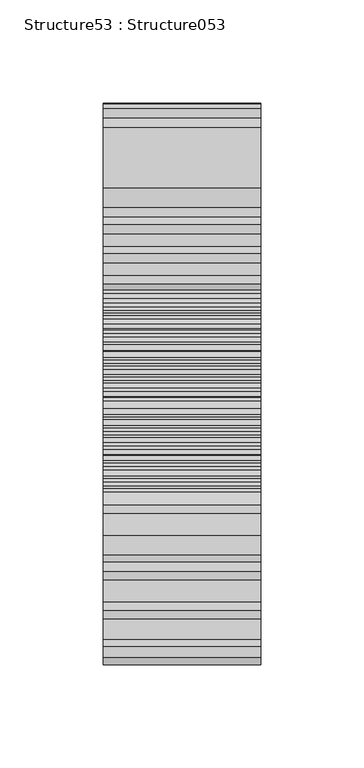
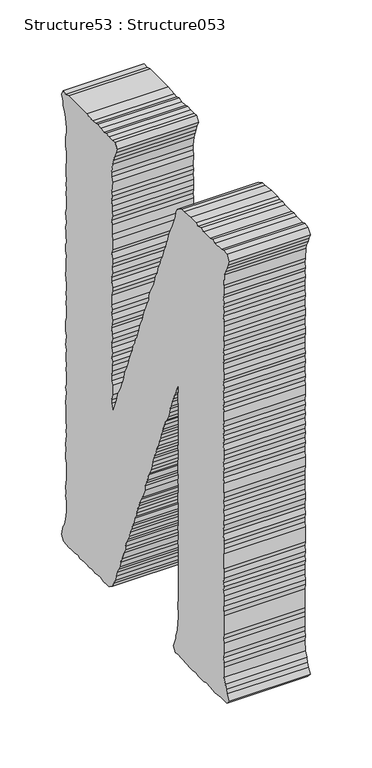
"""IFC4 building model written with IfcOpenShell, lengths in millimetres: proxy geometry, Structure53 : Structure053."""

from ifc_helpers import new_model, si_unit, frame, origin, place, context, project, spatial, polyline, outline, extrude, source, transform, mapped, element, save


def structure53_structure053_f29fcba1(model_context):
    return source(origin(), model_context, "Body", "SweptSolid", [
        extrude(outline(polyline([(256849.9794414, 3575.0851816), (256851.717228, 3569.2524442), (256852.3189547, 3565.7094775), (256855.839457, 3556.3417965), (256852.8982169, 3551.0658569), (256848.2175856, 3551.6675836), (256843.5385589, 3551.0658569), (256833.5755696, 3551.0658569), (256830.0550673, 3550.4833855), (256824.7727093, 3550.4833855), (256820.6954093, 3551.0658569), (256815.4130513, 3550.4833855), (256806.610191, 3550.4833855), (256802.508822, 3551.6675836), (256796.6696662, 3551.6675836), (256793.1266995, 3550.4833855), (256788.4685326, 3550.4833855), (256779.0864101, 3551.6675836), (256769.7042876, 3551.6675836), (256766.2046452, 3555.7416744), (256769.102561, 3561.025637), (256770.2835499, 3565.1254015), (256771.4645388, 3569.2524442), (256773.8040521, 3574.5107332), (256774.4057788, 3584.4689087), (256773.8040521, 3589.1527492), (256774.9866456, 3593.2541183), (256774.4057788, 3597.9540049), (256774.4057788, 3607.8961343), (256774.9866456, 3612.0135494), (256774.4057788, 3616.69739), (256774.4057788, 3635.4407751), (256773.8040521, 3640.114988), (256773.8040521, 3644.8245022), (256774.4057788, 3649.5003197), (256774.4057788, 3654.7842823), (256774.9866456, 3659.4584952), (256773.8040521, 3664.1423357), (256774.9866456, 3667.6853024), (256773.8040521, 3672.9435914), (256774.4057788, 3678.2018803), (256773.8040521, 3682.3289231), (256773.8040521, 3696.9709391), (256774.4057788, 3701.6547796), (256774.4057788, 3706.3289925), (256773.8040521, 3709.8559132), (256774.9866456, 3715.7143242), (256774.9866456, 3719.2316172), (256773.8040521, 3725.0996559), (256773.8040521, 3729.7738688), (256774.4057788, 3733.8736333), (256774.9866456, 3739.1592005), (256774.4057788, 3743.8414364), (256774.9866456, 3747.9428055), (256774.4057788, 3752.04257), (256773.8040521, 3757.3185096), (256773.8040521, 3766.684586), (256774.9866456, 3771.3860772), (256774.9866456, 3776.0618947), (256773.8040521, 3780.7441306), (256774.9866456, 3784.8438951), (256773.8040521, 3790.7039107), (256774.4057788, 3794.2292268), (256773.8040521, 3798.9050443), (256774.9866456, 3804.1890069), (256773.8040521, 3809.4729695), (256774.9866456, 3812.9726119), (256773.8040521, 3818.2309008), (256774.9866456, 3822.348316), (256773.8040521, 3828.2163546), (256773.8040521, 3837.6000817), (256774.9866456, 3841.6741725), (256773.8040521, 3846.3772683), (256774.9866456, 3851.0595042), (256774.9866456, 3855.1769193), (256773.8040521, 3861.0192843), (256774.9866456, 3865.7015202), (256773.8040521, 3869.2444869), (256774.4057788, 3873.9203044), (256774.9866456, 3879.1769888), (256774.9866456, 3884.4609514), (256773.8040521, 3888.5623205), (256773.8040521, 3893.822214), (256774.9866456, 3897.3475301), (256774.4057788, 3902.6314927), (256773.8040521, 3907.3313793), (256773.8040521, 3912.5896682), (256774.4057788, 3916.0909152), (256774.4057788, 3921.9733953), (256773.8040521, 3926.6492128), (256774.9866456, 3931.3346579), (256774.4057788, 3936.0345445), (256774.9866456, 3940.1166583), (256773.8040521, 3944.8165449), (256774.9866456, 3950.0940891), (256773.8040521, 3953.5937315), (256774.4057788, 3959.4617701), (256773.8040521, 3962.9774586), (256773.2247899, 3973.5197101), (256772.043801, 3977.6194746), (256769.102561, 3982.8793681), (256767.966501, 3986.4046842), (256766.2046452, 3991.0788971), (256769.7042876, 3996.390138), (256774.9866456, 3996.9645864), (256778.4846834, 3995.7803883), (256788.4685326, 3995.7803883), (256792.5474372, 3996.9645864), (256796.6696662, 3995.7803883), (256807.1894533, 3995.7803883), (256811.3116822, 3996.9645864), (256815.9923135, 3995.7803883), (256819.5144204, 3996.9645864), (256828.8965429, 3996.9645864), (256839.4371898, 3995.7803883), (256843.5385589, 3995.7803883), (256849.9794414, 3992.2614906), (256851.717228, 3988.7634528), (256852.8982169, 3982.8793681), (256854.6584681, 3978.8036727), (256856.4203238, 3974.7055128), (256857.6013127, 3971.1785921), (256860.5200883, 3966.5043792), (256862.2803394, 3961.2204166), (256864.0421952, 3957.1190475), (256865.2231841, 3952.9920048), (256867.540233, 3947.7337158), (256868.1419596, 3944.235678), (256870.481473, 3939.5325823), (256872.2433287, 3934.8503464), (256873.9811154, 3930.1745289), (256876.3430932, 3926.6492128), (256877.5240821, 3922.5494483), (256879.2859379, 3917.8479571), (256881.046189, 3914.3499193), (256882.2047134, 3909.0627475), (256885.123489, 3904.9645876), (256886.3060825, 3900.8648231), (256887.4870714, 3895.5888836), (256890.405847, 3890.905043), (256893.9279539, 3883.2863809), (256895.688205, 3879.1769888), (256896.2674672, 3874.5043805), (256898.6069806, 3869.8189354), (256900.3672317, 3864.5446004), (256902.7083497, 3860.4432313), (256903.8893386, 3857.5019912), (256905.6271253, 3851.6612309), (256906.8081142, 3848.7167816), (256909.1716966, 3844.0345457), (256910.9319477, 3838.7586061), (256912.0680077, 3834.6588416), (256913.8507233, 3830.5574726), (256915.0092477, 3825.2911606), (256917.9520924, 3822.348316), (256918.5313546, 3817.6741031), (256921.4501302, 3813.5743386), (256922.6311191, 3808.290376), (256924.9947015, 3803.5872802), (256926.7324882, 3799.5051664), (256928.4927393, 3795.4037973), (256929.0720015, 3791.8865042), (256931.435584, 3786.0280932), (256933.7750973, 3781.9299333), (256935.512884, 3777.8285642), (256936.6938729, 3773.11905), (256937.8748618, 3768.4432325), (256939.6367175, 3764.9435901), (256941.3969687, 3760.2437036), (256943.7140176, 3755.559863), (256946.0776, 3752.04257), (256948.4171133, 3743.2332913), (256950.1549, 3739.1592005), (256952.5168778, 3733.2991849), (256954.2787336, 3729.1737467), (256955.4597225, 3730.3563402), (256956.5957825, 3735.0578314), (256956.5957825, 3738.5574738), (256955.4597225, 3744.4158848), (256955.4597225, 3753.8012165), (256956.5957825, 3757.3185096), (256956.5957825, 3762.5848215), (256956.0389847, 3767.2590344), (256956.0389847, 3772.5606477), (256955.4597225, 3777.2444882), (256956.5957825, 3780.7441306), (256955.4597225, 3785.4456218), (256956.5957825, 3790.1294623), (256956.5957825, 3794.8309535), (256955.4597225, 3800.0876378), (256956.0389847, 3804.1890069), (256956.5957825, 3810.0474179), (256956.0389847, 3813.5743386), (256955.4597225, 3818.2309008), (256956.5957825, 3823.5341187), (256956.0389847, 3828.2163546), (256956.5957825, 3832.8921721), (256956.5957825, 3842.2758992), (256955.4597225, 3846.9757858), (256955.4597225, 3850.4754282), (256956.5957825, 3856.3161885), (256956.5957825, 3859.8591552), (256955.4597225, 3864.5446004), (256956.0389847, 3870.4030114), (256955.4597225, 3873.9203044), (256955.4597225, 3878.5784713), (256956.5957825, 3884.4609514), (256955.4597225, 3887.9621984), (256955.4597225, 3897.3475301), (256956.0389847, 3903.2059411), (256956.0389847, 3912.5896682), (256956.5957825, 3916.6653636), (256955.4597225, 3921.3748778), (256956.0389847, 3925.4746423), (256956.0389847, 3930.7329312), (256956.5957825, 3936.0345445), (256956.0389847, 3940.718385), (256956.5957825, 3944.235678), (256955.4597225, 3954.7506513), (256956.5957825, 3959.4617701), (256956.5957825, 3964.1343784), (256954.8579958, 3972.9372387), (256953.0977447, 3978.2035506), (256951.9151511, 3982.3225704), (256949.5756378, 3987.5792547), (256947.8378511, 3992.2614906), (256950.7566267, 3997.5486624), (256954.8579958, 3996.9645864), (256960.719616, 3996.9645864), (256965.3986427, 3997.5486624), (256968.9207496, 3996.390138), (256974.7807652, 3996.390138), (256979.4613965, 3997.5486624), (256982.9835034, 3996.390138), (256987.6625301, 3996.390138), (256997.0446526, 3997.5486624), (257026.3286846, 3997.5486624), (257031.0317804, 3996.390138), (257035.7124117, 3996.9645864), (257037.4726629, 3992.2614906), (257035.7124117, 3986.4046842), (257035.1331495, 3982.8793681), (257032.7695671, 3977.6194746), (257031.0317804, 3972.9372387), (257029.873256, 3962.9774586), (257029.873256, 3959.4617701), (257031.0317804, 3953.5937315), (257031.0317804, 3944.8165449), (257029.873256, 3940.1166583), (257029.873256, 3930.1745289), (257030.4525182, 3926.6492128), (257030.4525182, 3916.6653636), (257029.873256, 3912.0071968), (257030.4525182, 3907.3313793), (257029.873256, 3903.2059411), (257030.4525182, 3898.5301236), (257029.873256, 3893.246161), (257029.873256, 3883.8881076), (257031.0317804, 3879.1769888), (257029.873256, 3869.8189354), (257031.0317804, 3865.1190488), (257030.4525182, 3859.8591552), (257030.4525182, 3855.7353217), (257029.873256, 3850.4754282), (257031.0317804, 3846.9757858), (257031.0317804, 3841.0900965), (257029.873256, 3836.9919366), (257030.4525182, 3832.3161191), (257030.4525182, 3822.348316), (257031.0317804, 3818.2309008), (257030.4525182, 3812.9726119), (257029.873256, 3809.4729695), (257029.873256, 3804.7730829), (257030.4525182, 3799.5051664), (257029.873256, 3795.4037973), (257030.4525182, 3790.1294623), (257029.873256, 3784.8438951), (257029.873256, 3775.4874463), (257031.0317804, 3771.3860772), (257031.0317804, 3762.0023501), (257029.873256, 3757.8753073), (257030.4525182, 3752.04257), (257031.0317804, 3748.5429276), (257029.873256, 3743.8414364), (257030.4525182, 3739.1592005), (257030.4525182, 3734.47536), (257029.873256, 3728.5992983), (257030.4525182, 3725.0996559), (257029.873256, 3719.2316172), (257029.873256, 3709.8559132), (257031.0317804, 3705.7545441), (257029.873256, 3701.6547796), (257030.4525182, 3695.786741), (257031.0317804, 3691.0868544), (257030.4525182, 3687.0127636), (257030.4525182, 3672.3691429), (257029.873256, 3668.2437048), (257030.4525182, 3662.9854159), (257029.873256, 3659.4584952), (257030.4525182, 3653.6000842), (257031.0317804, 3650.1004418), (257030.4525182, 3644.2420307), (257031.0317804, 3640.114988), (257031.0317804, 3635.4407751), (257029.873256, 3631.3410106), (257029.873256, 3616.69739), (257030.4525182, 3611.4134274), (257031.0317804, 3607.3393366), (257030.4525182, 3602.0280957), (257031.0317804, 3598.5284533), (257029.873256, 3593.2541183), (257029.873256, 3583.2863152), (257031.0317804, 3575.0851816), (257032.7695671, 3569.2524442), (257035.1331495, 3565.7094775), (257036.8934006, 3559.8671125), (257038.0743895, 3556.3417965), (257034.5522827, 3551.0658569), (257030.4525182, 3551.0658569), (257026.3286846, 3550.4833855), (257020.4911335, 3551.0658569), (257016.3897644, 3551.0658569), (257011.1074064, 3551.6675836), (257007.6093686, 3550.4833855), (257001.7252839, 3551.0658569), (256998.2272461, 3551.0658569), (256992.3656259, 3550.4833855), (256988.2417923, 3551.6675836), (256983.5627656, 3550.4833855), (256978.3028721, 3551.6675836), (256974.7807652, 3551.6675836), (256970.1017385, 3550.4833855), (256964.8193805, 3551.0658569), (256960.719616, 3551.0658569), (256954.8579958, 3555.1848766), (256953.0977447, 3559.2669905), (256950.1549, 3563.9412034), (256949.5756378, 3568.0682461), (256947.8378511, 3573.3265351), (256945.4758733, 3577.4535778), (256943.1347553, 3581.5276686), (256941.9537664, 3586.8116312), (256939.6367175, 3591.5131224), (256936.1146107, 3599.7126514), (256934.3318951, 3603.7963698), (256933.7750973, 3607.3393366), (256932.0148462, 3613.1720739), (256930.2529905, 3616.69739), (256927.3117504, 3621.3732075), (256926.7324882, 3625.472972), (256924.3929748, 3630.1824862), (256922.6311191, 3634.2822506), (256920.2916057, 3638.3563415), (256919.6898791, 3643.6579547), (256917.3728302, 3647.1575971), (256915.0092477, 3651.8590883), (256914.4299855, 3655.9428067), (256912.0680077, 3660.6250426), (256910.9319477, 3664.1423357), (256909.1716966, 3668.8261762), (256906.2288519, 3672.9435914), (256902.7083497, 3681.7271964), (256902.1290875, 3686.4030139), (256899.7879695, 3691.0868544), (256898.0277184, 3694.6298211), (256896.8467295, 3700.4705815), (256895.1089428, 3703.4134261), (256892.7453604, 3708.087639), (256890.9851092, 3712.7971532), (256890.405847, 3716.8985223), (256888.6680603, 3722.1568112), (256886.9078092, 3725.6741043), (256884.5442268, 3730.3563402), (256883.3632379, 3733.8736333), (256880.4444623, 3739.1592005), (256879.8652001, 3743.8414364), (256877.5240821, 3748.5429276), (256876.3430932, 3752.6170184), (256873.9811154, 3757.3185096), (256872.8450554, 3760.2437036), (256870.481473, 3766.1021146), (256869.3004841, 3770.2018791), (256866.404173, 3773.7015215), (256864.6439218, 3777.8285642), (256862.8596016, 3782.5027771), (256861.7010772, 3787.2042683), (256860.5200883, 3790.7039107), (256858.7823016, 3795.960595), (256855.839457, 3800.6717138), (256854.6584681, 3804.7730829), (256852.8982169, 3808.290376), (256851.1604303, 3812.9726119), (256848.8193123, 3817.6741031), (256847.6383234, 3818.2309008), (256848.2175856, 3812.9726119), (256848.8193123, 3808.8888934), (256848.8193123, 3803.0064134), (256848.2175856, 3798.9050443), (256847.6383234, 3794.2292268), (256848.2175856, 3790.1294623), (256848.2175856, 3780.7441306), (256847.6383234, 3774.8857196), (256847.6383234, 3766.684586), (256848.2175856, 3760.818152), (256848.8193123, 3757.3185096), (256848.2175856, 3752.6170184), (256847.6383234, 3747.3587295), (256848.8193123, 3742.6748889), (256848.8193123, 3732.7167134), (256848.2175856, 3728.0152223), (256848.8193123, 3723.9154578), (256848.2175856, 3718.6571688), (256847.6383234, 3714.5301261), (256848.8193123, 3709.8559132), (256848.8193123, 3704.5879966), (256848.2175856, 3700.4705815), (256847.6383234, 3696.3884676), (256847.6383234, 3691.6869765), (256848.2175856, 3687.587212), (256848.2175856, 3681.7271964), (256848.8193123, 3677.0449605), (256848.2175856, 3672.3691429), (256847.6383234, 3668.2437048), (256848.8193123, 3663.5598643), (256847.6383234, 3658.3015753), (256847.6383234, 3648.9258713), (256848.2175856, 3644.8245022), (256848.2175856, 3635.4407751), (256847.6383234, 3631.3410106), (256847.6383234, 3611.4134274), (256848.2175856, 3607.3393366), (256848.8193123, 3602.0280957), (256848.8193123, 3597.9540049), (256847.6383234, 3593.8285667), (256847.6383234, 3589.1527492), (256848.8193123, 3583.2863152), (256849.9794414, 3575.0851816)])), frame((-38594.2176606, 0.0, 0.0), z_axis=(1.0, 0.0, 0.0), x_axis=(0.0, 1.0, 0.0)), (0.0, 0.0, 1.0), 76.2),
    ])


if __name__ == "__main__":
    model = new_model("IFC4")
    model_context = context("Model", 3, world=origin())
    ifc_project = project(units=[si_unit("LENGTHUNIT", "METRE", prefix="MILLI")], contexts=[model_context])
    site = spatial("IfcSite", under=ifc_project)
    building = spatial("IfcBuilding", under=site)
    placement = place(None, origin())
    structure53_structure053_shape = structure53_structure053_f29fcba1(model_context)
    element("IfcBuildingElementProxy", 1, Name="Structure53 : Structure053", ObjectType="Structure53 : Structure053", at=placement, inside=building, context=model_context, shape_type="MappedRepresentation", body=[
        mapped(structure53_structure053_shape, transform((0.0, 0.0, 0.0), x_axis=(1.0, 0.0, 0.0), y_axis=(0.0, 1.0, 0.0), z_axis=(0.0, 0.0, 1.0))),
    ])
    save(model, "model.ifc")

# Revit data of these elements
# Type "Structure53 : Structure053"
#   NameOverride = "Structure053"
# Element 1 (IfcBuildingElementProxy, "Structure53 : Structure053")
#   Materials on its faces: "BRUSHED ALUM. LETTERING"
# Materials
#   "BRUSHED ALUM. LETTERING": class "Unassigned", colour RGB 169 181 186, transparency 0, Cost = 0
